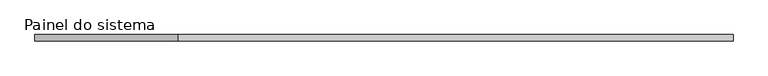
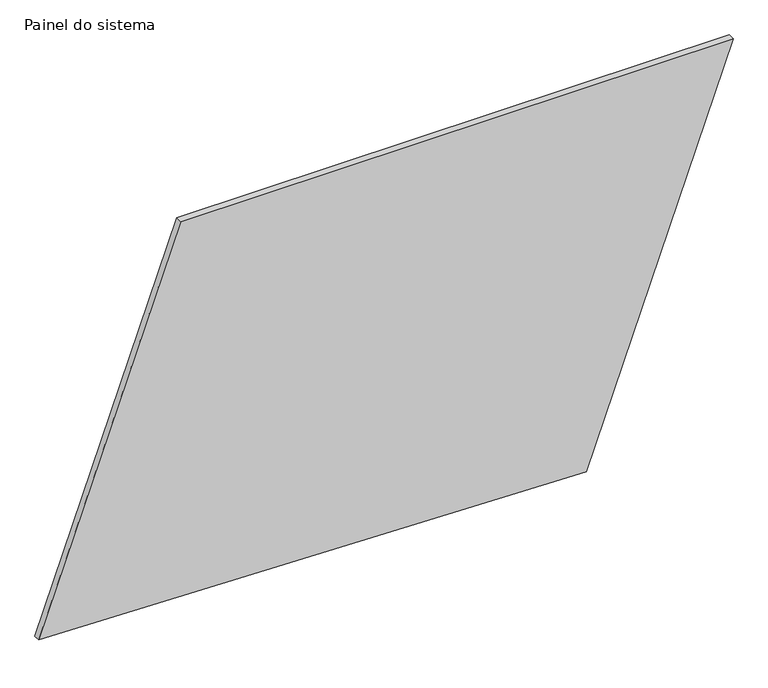
"""IFC4 building model written with IfcOpenShell, lengths in millimetres: plate geometry, Painel do sistema : Envidraçado."""

from ifc_helpers import new_model, si_unit, frame, origin, place, context, project, spatial, polyline, outline, extrude, source, transform, mapped, element, save


def painel_do_sistema_03db7a64(model_context):
    return source(origin(), model_context, "Body", "SweptSolid", [
        extrude(outline(polyline([(56.0236852, -1377.9540601), (0.0, 794.4180475), (1612.9566656, 1377.9540601), (1612.9566656, -814.6863155), (56.0236852, -1377.9540601)])), frame((0.0, 24.5, 0.0), z_axis=(0.0, 1.0, 0.0), x_axis=(0.0, 0.0, 1.0)), (0.0, 0.0, 1.0), 25.0),
    ])


if __name__ == "__main__":
    model = new_model("IFC4")
    model_context = context("Model", 3, world=origin())
    ifc_project = project(units=[si_unit("LENGTHUNIT", "METRE", prefix="MILLI")], contexts=[model_context])
    site = spatial("IfcSite", under=ifc_project)
    building = spatial("IfcBuilding", under=site)
    placement = place(None, origin())
    painel_do_sistema_shape = painel_do_sistema_03db7a64(model_context)
    element("IfcPlate", 1, ObjectType="Painel do sistema : Envidraçado", at=placement, inside=building, context=model_context, shape_type="MappedRepresentation", body=[
        mapped(painel_do_sistema_shape, transform((0.0, 0.0, 0.0), x_axis=(1.0, 0.0, 0.0), y_axis=(0.0, 1.0, 0.0), z_axis=(0.0, 0.0, 1.0))),
    ])
    save(model, "model.ifc")

# Revit data of these elements
# Type "Painel do sistema : Envidraçado"
#   Construction Type Id = "GSP4R"
#   Analytic Construction = "Vidraça única Pilkington 1/8 pol"
#   Visual Light Transmittance = 0.9
#   Solar Heat Gain Coefficient = 0.86
#   Heat Transfer Coefficient (U) = 6.7069 W/(m²·K)
# Element 1 (IfcPlate, "Painel do sistema : Envidraçado")
#   Materials on its faces: "Vidro"
# Materials
#   "Vidro": class "Vidro", colour RGB 0 128 192, transparency 0.9, Description = "Vidro de sílica", Cost = 0
